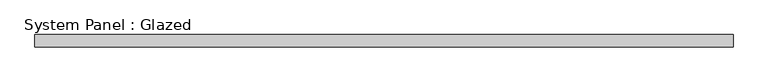
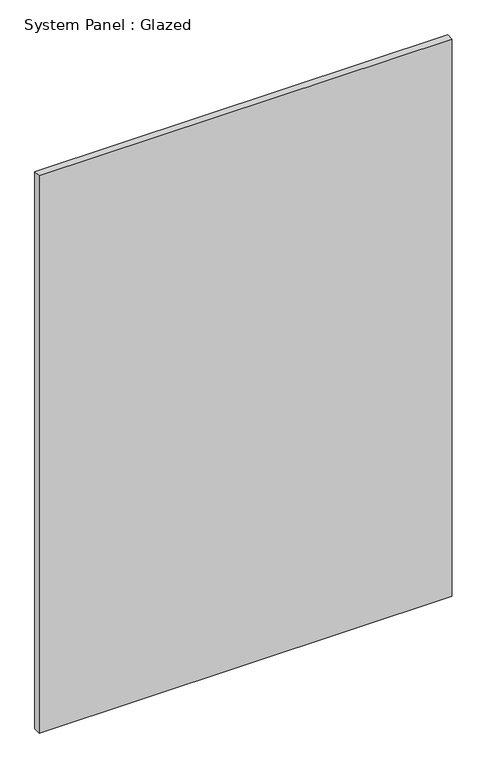
"""IFC4 building model written with IfcOpenShell, lengths in millimetres: plate geometry, System Panel : Glazed."""

from ifc_helpers import new_model, si_unit, origin, origin_with_axes, place, context, project, spatial, polyline, outline, extrude, source, transform, mapped, element, save


def system_panel_glazed_60c4151f(model_context):
    return source(origin(), model_context, "Body", "SweptSolid", [
        extrude(outline(polyline([(712.5000001, 24.5), (-712.5000001, 24.5), (-712.5000001, 49.5), (712.5000001, 49.5), (712.5000001, 24.5)])), origin_with_axes(), (0.0, 0.0, 1.0), 2030.4462072),
    ])


if __name__ == "__main__":
    model = new_model("IFC4")
    model_context = context("Model", 3, world=origin())
    ifc_project = project(units=[si_unit("LENGTHUNIT", "METRE", prefix="MILLI")], contexts=[model_context])
    site = spatial("IfcSite", under=ifc_project)
    building = spatial("IfcBuilding", under=site)
    placement = place(None, origin())
    system_panel_glazed_shape = system_panel_glazed_60c4151f(model_context)
    element("IfcPlate", 1, ObjectType="System Panel : Glazed", at=placement, inside=building, context=model_context, shape_type="MappedRepresentation", body=[
        mapped(system_panel_glazed_shape, transform((0.0, 0.0, 0.0), x_axis=(1.0, 0.0, 0.0), y_axis=(0.0, 1.0, 0.0), z_axis=(0.0, 0.0, 1.0))),
    ])
    save(model, "model.ifc")

# Revit data of these elements
# Type "System Panel : Glazed"
#   Construction Type Id = "GSP4R"
#   Analytic Construction = "1/8 in Pilkington single glazing"
#   Visual Light Transmittance = 0.9
#   Solar Heat Gain Coefficient = 0.86
#   Heat Transfer Coefficient (U) = 6.7069 W/(m²·K)
#   Define Thermal Properties by = 1
# Element 1 (IfcPlate, "System Panel : Glazed")
#   Materials on its faces: "Glass"
# Materials
#   "Glass": class "Glass", colour RGB 0 128 192, transparency 0.9, Description = "Soda Lime Glass", Cost = 0
